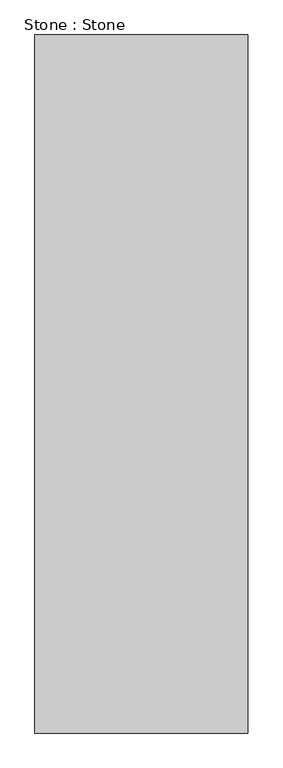
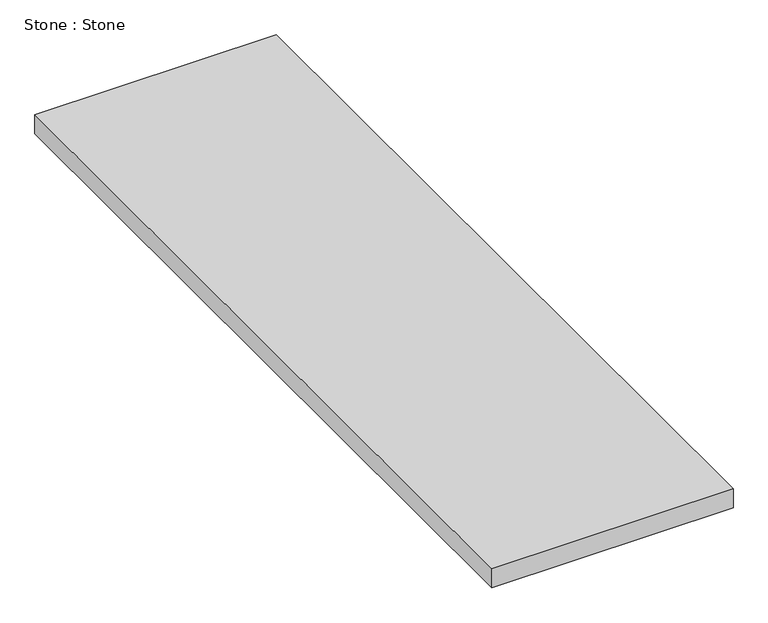
"""IFC4 building model written with IfcOpenShell, lengths in millimetres: proxy geometry, Stone : Stone."""

import ifcopenshell
import ifcopenshell.guid

model = None  # the IFC model being written
_history = None  # IfcOwnerHistory: only IFC2X3 demands one
_inside = {}  # id of a spatial element -> (the spatial element, [elements in it])
_under = {}  # id of a project, library or spatial element -> (it, [spatial elements below it])
_declared = {}  # id of a project -> (the project, [libraries it declares])
_typed = {}  # id of a type object -> (the type object, [elements of that type])
_made_of = {}  # id of a material, layer set ... -> (it, [elements and type objects made of it])


def new_model(schema):
    """Start an empty IFC model of exactly this schema.

    Asked for "IFC4X3", IfcOpenShell would pick the latest addendum, in which some entities
    have other attributes; the version numbers below select the first issue.
    IFC2X3 requires an IfcOwnerHistory on every rooted entity: one is made here for all.
    """
    global model, _history
    if schema == "IFC4X3":
        model = ifcopenshell.file(schema_version=(4, 3, 0, 0))
    else:
        model = ifcopenshell.file(schema=schema)
    _inside.clear()
    _under.clear()
    _declared.clear()
    _typed.clear()
    _made_of.clear()
    _history = None
    if model.schema == "IFC2X3":
        org = make("IfcOrganization", Name="unknown")
        user = make(
            "IfcPersonAndOrganization",
            ThePerson=make("IfcPerson", FamilyName="unknown"),
            TheOrganization=org,
        )
        app = make(
            "IfcApplication",
            ApplicationDeveloper=org,
            Version="unknown",
            ApplicationFullName="unknown",
            ApplicationIdentifier="unknown",
        )
        _history = make(
            "IfcOwnerHistory",
            OwningUser=user,
            OwningApplication=app,
            ChangeAction="ADDED",
            CreationDate=0,
        )
    return model


def make(cls, **values):
    """One entity of the class cls with the attributes given. An attribute that is None is left unset."""
    return model.create_entity(
        cls, **{name: value for name, value in values.items() if value is not None}
    )


def rooted(cls, **values):
    """An entity with a GlobalId (a new one), such as an element, a storey or a relation."""
    return make(cls, GlobalId=ifcopenshell.guid.new(), OwnerHistory=_history, **values)


def si_unit(unit_type, name, prefix=None):
    """IfcSIUnit, for example si_unit("LENGTHUNIT", "METRE", prefix="MILLI")."""
    return make("IfcSIUnit", UnitType=unit_type, Prefix=prefix, Name=name)


def assignment(units):
    """IfcUnitAssignment: the units of a project."""
    return None if units is None else make("IfcUnitAssignment", Units=units)


def point(xyz):
    """IfcCartesianPoint."""
    return None if xyz is None else make("IfcCartesianPoint", Coordinates=xyz)


def direction(xyz):
    """IfcDirection."""
    return None if xyz is None else make("IfcDirection", DirectionRatios=xyz)


def frame(location, z_axis=None, x_axis=None):
    """IfcAxis2Placement3D, a coordinate frame: its origin and axes. An axis left out is left unset."""
    return make(
        "IfcAxis2Placement3D",
        Location=point(location),
        Axis=direction(z_axis),
        RefDirection=direction(x_axis),
    )


def origin():
    """The frame at (0, 0, 0) with its axes left unset."""
    return frame((0.0, 0.0, 0.0))


def place(relative_to, where):
    """IfcLocalPlacement: puts the frame where relative to a parent placement (None: the world)."""
    return make(
        "IfcLocalPlacement", PlacementRelTo=relative_to, RelativePlacement=where
    )


def context(
    kind, dimensions, precision=None, world=None, true_north=None, identifier=None
):
    """IfcGeometricRepresentationContext, for example the 3D "Model" context."""
    return make(
        "IfcGeometricRepresentationContext",
        ContextIdentifier=identifier,
        ContextType=kind,
        CoordinateSpaceDimension=dimensions,
        Precision=precision,
        WorldCoordinateSystem=world,
        TrueNorth=true_north,
    )


def project(units=None, contexts=None):
    """IfcProject with its units and contexts."""
    return rooted(
        "IfcProject",
        Name="project",
        RepresentationContexts=contexts,
        UnitsInContext=assignment(units),
    )


def spatial(cls, under=None, at=None, **own):
    """A site, building, storey or space (cls), placed at a placement, below another one or the project."""
    s = rooted(cls, ObjectPlacement=at, **own)
    if under is not None:
        _under.setdefault(under.id(), (under, []))[1].append(s)
    return s


def polyline(points):
    """IfcPolyline through the points."""
    return make("IfcPolyline", Points=[point(p) for p in points])


def outline(outer, holes=None, kind="AREA"):
    """IfcArbitraryClosedProfileDef: a profile drawn as a closed curve; with holes, ...WithVoids."""
    if holes is None:
        return make("IfcArbitraryClosedProfileDef", ProfileType=kind, OuterCurve=outer)
    return make(
        "IfcArbitraryProfileDefWithVoids",
        ProfileType=kind,
        OuterCurve=outer,
        InnerCurves=holes,
    )


def extrude(swept, where, along, depth):
    """IfcExtrudedAreaSolid: the profile swept, set in the frame where, extruded along a direction by depth."""
    return make(
        "IfcExtrudedAreaSolid",
        SweptArea=swept,
        Position=where,
        ExtrudedDirection=direction(along),
        Depth=depth,
    )


def shape(context_of_items, identifier, shape_type, items):
    """IfcShapeRepresentation: the items that make up one representation, for example the "Body"."""
    return make(
        "IfcShapeRepresentation",
        ContextOfItems=context_of_items,
        RepresentationIdentifier=identifier,
        RepresentationType=shape_type,
        Items=items,
    )


def source(mapping_origin, context_of_items, identifier, shape_type, items):
    """IfcRepresentationMap: a shape defined once, which mapped items show again and again."""
    return make(
        "IfcRepresentationMap",
        MappingOrigin=mapping_origin,
        MappedRepresentation=shape(context_of_items, identifier, shape_type, items),
    )


def transform(
    local_origin,
    x_axis=None,
    y_axis=None,
    z_axis=None,
    scale=None,
    scale2=None,
    scale3=None,
    uniform=True,
):
    """IfcCartesianTransformationOperator3D, or its non-uniform kind. x_axis, y_axis, z_axis: its Axis1, 2, 3."""
    if uniform:
        return make(
            "IfcCartesianTransformationOperator3D",
            Axis1=direction(x_axis),
            Axis2=direction(y_axis),
            LocalOrigin=point(local_origin),
            Scale=scale,
            Axis3=direction(z_axis),
        )
    return make(
        "IfcCartesianTransformationOperator3DnonUniform",
        Axis1=direction(x_axis),
        Axis2=direction(y_axis),
        LocalOrigin=point(local_origin),
        Scale=scale,
        Axis3=direction(z_axis),
        Scale2=scale2,
        Scale3=scale3,
    )


def mapped(mapping_source, mapping_target):
    """IfcMappedItem: shows the shape of a source again, moved by a transform."""
    return make(
        "IfcMappedItem", MappingSource=mapping_source, MappingTarget=mapping_target
    )


def made_of(thing, what):
    """Note that an element or type object is made of a material, layer set ...; save() writes the relation."""
    if what is not None:
        _made_of.setdefault(what.id(), (what, []))[1].append(thing)
    return thing


def element(
    cls,
    number,
    at=None,
    inside=None,
    cuts=None,
    type_object=None,
    material=None,
    context=None,
    identifier="Body",
    shape_type=None,
    held_by="IfcProductDefinitionShape",
    body=None,
    shapes=None,
    **own,
):
    """One element of the class cls, such as IfcWall. Its Tag is "e" and its number.

    at: its placement. inside: the storey or other place that contains it. cuts: it is an
    opening in that element (IfcRelVoidsElement). A single representation is given by context,
    identifier, shape_type and body (its items); several are given by shapes. held_by: the class
    of the entity that holds the representations. save() writes the other relations.
    """
    e = rooted(cls, Tag="e%d" % number, ObjectPlacement=at, **own)
    if body is not None:
        shapes = [shape(context, identifier, shape_type, body)]
    if shapes is not None:
        e.Representation = make(held_by, Representations=shapes)
    if inside is not None:
        _inside.setdefault(inside.id(), (inside, []))[1].append(e)
    if cuts is not None:
        rooted(
            "IfcRelVoidsElement", RelatingBuildingElement=cuts, RelatedOpeningElement=e
        )
    if type_object is not None:
        _typed.setdefault(type_object.id(), (type_object, []))[1].append(e)
    return made_of(e, material)


def aggregate(whole, parts):
    """IfcRelAggregates: a whole, such as a stair, and the parts it consists of."""
    return rooted("IfcRelAggregates", RelatingObject=whole, RelatedObjects=parts)


def save(model, path):
    """Write the relations noted so far, then the file.

    IfcRelAggregates (storeys below a building ...), IfcRelContainedInSpatialStructure (elements
    in a storey), IfcRelDefinesByType, IfcRelAssociatesMaterial and IfcRelDeclares: one each for
    every whole, place, type object, material and project.
    """
    for whole, parts in _under.values():
        aggregate(whole, parts)
    for where, things in _inside.values():
        rooted(
            "IfcRelContainedInSpatialStructure",
            RelatedElements=things,
            RelatingStructure=where,
        )
    for kind, things in _typed.values():
        rooted("IfcRelDefinesByType", RelatedObjects=things, RelatingType=kind)
    for what, things in _made_of.values():
        rooted("IfcRelAssociatesMaterial", RelatedObjects=things, RelatingMaterial=what)
    for by, libraries in _declared.values():
        rooted("IfcRelDeclares", RelatingContext=by, RelatedDefinitions=libraries)
    model.write(path)


def stone_stone_c53325bf(model_context):
    return source(origin(), model_context, "Body", "SweptSolid", [
        extrude(outline(polyline([(-5504.8492306, -1052.8906574), (-6114.4492306, -1052.8906574), (-6114.4492306, 947.1093426), (-5504.8492306, 947.1093426), (-5504.8492306, -1052.8906574)])), frame((0.0, 0.0, 36508.2444375), z_axis=(0.0, 0.0, 1.0), x_axis=(1.0, 0.0, 0.0)), (0.0, 0.0, 1.0), 50.8),
    ])


if __name__ == "__main__":
    model = new_model("IFC4")
    model_context = context("Model", 3, world=origin())
    ifc_project = project(units=[si_unit("LENGTHUNIT", "METRE", prefix="MILLI")], contexts=[model_context])
    site = spatial("IfcSite", under=ifc_project)
    building = spatial("IfcBuilding", under=site)
    placement = place(None, origin())
    stone_stone_shape = stone_stone_c53325bf(model_context)
    element("IfcBuildingElementProxy", 1, Name="Stone : Stone", ObjectType="Stone : Stone", at=placement, inside=building, context=model_context, shape_type="MappedRepresentation", body=[
        mapped(stone_stone_shape, transform((0.0, 0.0, 0.0), x_axis=(1.0, 0.0, 0.0), y_axis=(0.0, 1.0, 0.0), z_axis=(0.0, 0.0, 1.0))),
    ])
    save(model, "model.ifc")

# Revit data of these elements
# Type "Stone : Stone"
#   NameOverride = "Stone"
# Element 1 (IfcBuildingElementProxy, "Stone : Stone")
#   Materials on its faces: "2\" STONE DECK TBD"
# Materials
#   "2\" STONE DECK TBD": class "Unassigned", colour RGB 199 185 173, transparency 0
